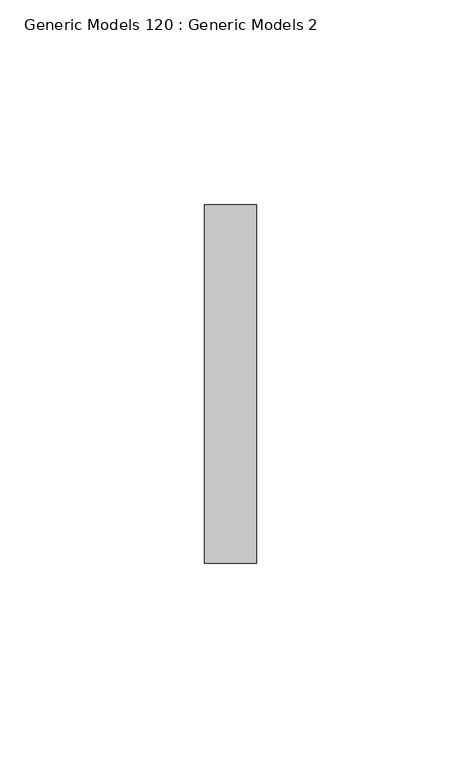
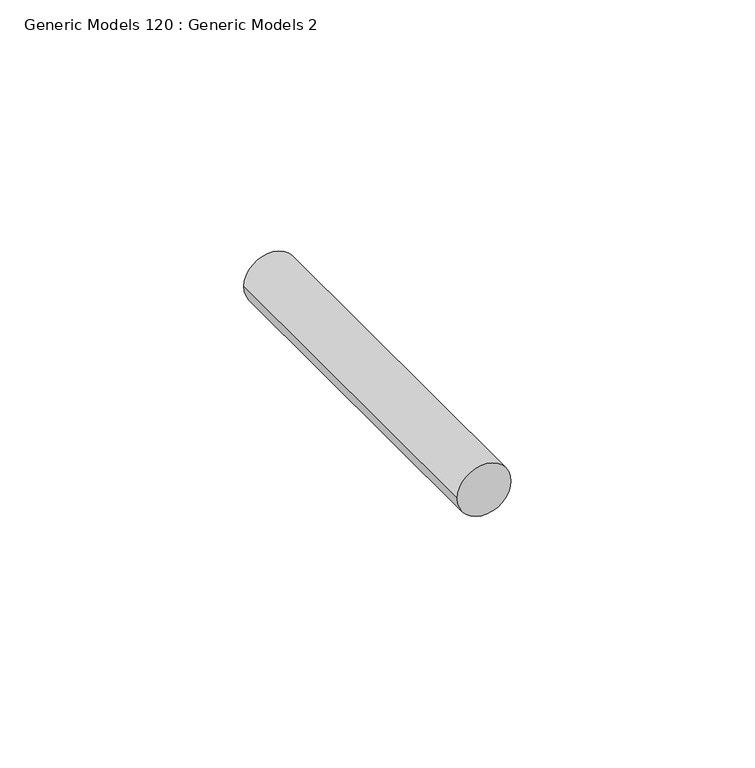
"""IFC4 building model written with IfcOpenShell, lengths in millimetres: proxy geometry, Generic Models 120 : Generic Models 2."""

import ifcopenshell
import ifcopenshell.guid

model = None  # the IFC model being written
_history = None  # IfcOwnerHistory: only IFC2X3 demands one
_inside = {}  # id of a spatial element -> (the spatial element, [elements in it])
_under = {}  # id of a project, library or spatial element -> (it, [spatial elements below it])
_declared = {}  # id of a project -> (the project, [libraries it declares])
_typed = {}  # id of a type object -> (the type object, [elements of that type])
_made_of = {}  # id of a material, layer set ... -> (it, [elements and type objects made of it])


def new_model(schema):
    """Start an empty IFC model of exactly this schema.

    Asked for "IFC4X3", IfcOpenShell would pick the latest addendum, in which some entities
    have other attributes; the version numbers below select the first issue.
    IFC2X3 requires an IfcOwnerHistory on every rooted entity: one is made here for all.
    """
    global model, _history
    if schema == "IFC4X3":
        model = ifcopenshell.file(schema_version=(4, 3, 0, 0))
    else:
        model = ifcopenshell.file(schema=schema)
    _inside.clear()
    _under.clear()
    _declared.clear()
    _typed.clear()
    _made_of.clear()
    _history = None
    if model.schema == "IFC2X3":
        org = make("IfcOrganization", Name="unknown")
        user = make(
            "IfcPersonAndOrganization",
            ThePerson=make("IfcPerson", FamilyName="unknown"),
            TheOrganization=org,
        )
        app = make(
            "IfcApplication",
            ApplicationDeveloper=org,
            Version="unknown",
            ApplicationFullName="unknown",
            ApplicationIdentifier="unknown",
        )
        _history = make(
            "IfcOwnerHistory",
            OwningUser=user,
            OwningApplication=app,
            ChangeAction="ADDED",
            CreationDate=0,
        )
    return model


def make(cls, **values):
    """One entity of the class cls with the attributes given. An attribute that is None is left unset."""
    return model.create_entity(
        cls, **{name: value for name, value in values.items() if value is not None}
    )


def rooted(cls, **values):
    """An entity with a GlobalId (a new one), such as an element, a storey or a relation."""
    return make(cls, GlobalId=ifcopenshell.guid.new(), OwnerHistory=_history, **values)


def si_unit(unit_type, name, prefix=None):
    """IfcSIUnit, for example si_unit("LENGTHUNIT", "METRE", prefix="MILLI")."""
    return make("IfcSIUnit", UnitType=unit_type, Prefix=prefix, Name=name)


def assignment(units):
    """IfcUnitAssignment: the units of a project."""
    return None if units is None else make("IfcUnitAssignment", Units=units)


def point(xyz):
    """IfcCartesianPoint."""
    return None if xyz is None else make("IfcCartesianPoint", Coordinates=xyz)


def direction(xyz):
    """IfcDirection."""
    return None if xyz is None else make("IfcDirection", DirectionRatios=xyz)


def frame(location, z_axis=None, x_axis=None):
    """IfcAxis2Placement3D, a coordinate frame: its origin and axes. An axis left out is left unset."""
    return make(
        "IfcAxis2Placement3D",
        Location=point(location),
        Axis=direction(z_axis),
        RefDirection=direction(x_axis),
    )


def frame_2d(location, x_axis=None):
    """IfcAxis2Placement2D, a coordinate frame in the plane: its origin and x axis."""
    return make(
        "IfcAxis2Placement2D", Location=point(location), RefDirection=direction(x_axis)
    )


def origin():
    """The frame at (0, 0, 0) with its axes left unset."""
    return frame((0.0, 0.0, 0.0))


def place(relative_to, where):
    """IfcLocalPlacement: puts the frame where relative to a parent placement (None: the world)."""
    return make(
        "IfcLocalPlacement", PlacementRelTo=relative_to, RelativePlacement=where
    )


def context(
    kind, dimensions, precision=None, world=None, true_north=None, identifier=None
):
    """IfcGeometricRepresentationContext, for example the 3D "Model" context."""
    return make(
        "IfcGeometricRepresentationContext",
        ContextIdentifier=identifier,
        ContextType=kind,
        CoordinateSpaceDimension=dimensions,
        Precision=precision,
        WorldCoordinateSystem=world,
        TrueNorth=true_north,
    )


def project(units=None, contexts=None):
    """IfcProject with its units and contexts."""
    return rooted(
        "IfcProject",
        Name="project",
        RepresentationContexts=contexts,
        UnitsInContext=assignment(units),
    )


def spatial(cls, under=None, at=None, **own):
    """A site, building, storey or space (cls), placed at a placement, below another one or the project."""
    s = rooted(cls, ObjectPlacement=at, **own)
    if under is not None:
        _under.setdefault(under.id(), (under, []))[1].append(s)
    return s


def circle_curve(where, radius):
    """IfcCircle in the frame where."""
    return make("IfcCircle", Position=where, Radius=radius)


def trimmed(basis, trim1, trim2, sense, master):
    """IfcTrimmedCurve: the piece of a basis curve between two trims."""
    return make(
        "IfcTrimmedCurve",
        BasisCurve=basis,
        Trim1=trim1,
        Trim2=trim2,
        SenseAgreement=sense,
        MasterRepresentation=master,
    )


def segment(curve, same_sense, transition):
    """IfcCompositeCurveSegment."""
    return make(
        "IfcCompositeCurveSegment",
        Transition=transition,
        SameSense=same_sense,
        ParentCurve=curve,
    )


def composite_curve(segments, self_intersect=None):
    """IfcCompositeCurve: segments joined end to end."""
    return make("IfcCompositeCurve", Segments=segments, SelfIntersect=self_intersect)


def outline(outer, holes=None, kind="AREA"):
    """IfcArbitraryClosedProfileDef: a profile drawn as a closed curve; with holes, ...WithVoids."""
    if holes is None:
        return make("IfcArbitraryClosedProfileDef", ProfileType=kind, OuterCurve=outer)
    return make(
        "IfcArbitraryProfileDefWithVoids",
        ProfileType=kind,
        OuterCurve=outer,
        InnerCurves=holes,
    )


def extrude(swept, where, along, depth):
    """IfcExtrudedAreaSolid: the profile swept, set in the frame where, extruded along a direction by depth."""
    return make(
        "IfcExtrudedAreaSolid",
        SweptArea=swept,
        Position=where,
        ExtrudedDirection=direction(along),
        Depth=depth,
    )


def shape(context_of_items, identifier, shape_type, items):
    """IfcShapeRepresentation: the items that make up one representation, for example the "Body"."""
    return make(
        "IfcShapeRepresentation",
        ContextOfItems=context_of_items,
        RepresentationIdentifier=identifier,
        RepresentationType=shape_type,
        Items=items,
    )


def source(mapping_origin, context_of_items, identifier, shape_type, items):
    """IfcRepresentationMap: a shape defined once, which mapped items show again and again."""
    return make(
        "IfcRepresentationMap",
        MappingOrigin=mapping_origin,
        MappedRepresentation=shape(context_of_items, identifier, shape_type, items),
    )


def transform(
    local_origin,
    x_axis=None,
    y_axis=None,
    z_axis=None,
    scale=None,
    scale2=None,
    scale3=None,
    uniform=True,
):
    """IfcCartesianTransformationOperator3D, or its non-uniform kind. x_axis, y_axis, z_axis: its Axis1, 2, 3."""
    if uniform:
        return make(
            "IfcCartesianTransformationOperator3D",
            Axis1=direction(x_axis),
            Axis2=direction(y_axis),
            LocalOrigin=point(local_origin),
            Scale=scale,
            Axis3=direction(z_axis),
        )
    return make(
        "IfcCartesianTransformationOperator3DnonUniform",
        Axis1=direction(x_axis),
        Axis2=direction(y_axis),
        LocalOrigin=point(local_origin),
        Scale=scale,
        Axis3=direction(z_axis),
        Scale2=scale2,
        Scale3=scale3,
    )


def mapped(mapping_source, mapping_target):
    """IfcMappedItem: shows the shape of a source again, moved by a transform."""
    return make(
        "IfcMappedItem", MappingSource=mapping_source, MappingTarget=mapping_target
    )


def made_of(thing, what):
    """Note that an element or type object is made of a material, layer set ...; save() writes the relation."""
    if what is not None:
        _made_of.setdefault(what.id(), (what, []))[1].append(thing)
    return thing


def element(
    cls,
    number,
    at=None,
    inside=None,
    cuts=None,
    type_object=None,
    material=None,
    context=None,
    identifier="Body",
    shape_type=None,
    held_by="IfcProductDefinitionShape",
    body=None,
    shapes=None,
    **own,
):
    """One element of the class cls, such as IfcWall. Its Tag is "e" and its number.

    at: its placement. inside: the storey or other place that contains it. cuts: it is an
    opening in that element (IfcRelVoidsElement). A single representation is given by context,
    identifier, shape_type and body (its items); several are given by shapes. held_by: the class
    of the entity that holds the representations. save() writes the other relations.
    """
    e = rooted(cls, Tag="e%d" % number, ObjectPlacement=at, **own)
    if body is not None:
        shapes = [shape(context, identifier, shape_type, body)]
    if shapes is not None:
        e.Representation = make(held_by, Representations=shapes)
    if inside is not None:
        _inside.setdefault(inside.id(), (inside, []))[1].append(e)
    if cuts is not None:
        rooted(
            "IfcRelVoidsElement", RelatingBuildingElement=cuts, RelatedOpeningElement=e
        )
    if type_object is not None:
        _typed.setdefault(type_object.id(), (type_object, []))[1].append(e)
    return made_of(e, material)


def aggregate(whole, parts):
    """IfcRelAggregates: a whole, such as a stair, and the parts it consists of."""
    return rooted("IfcRelAggregates", RelatingObject=whole, RelatedObjects=parts)


def save(model, path):
    """Write the relations noted so far, then the file.

    IfcRelAggregates (storeys below a building ...), IfcRelContainedInSpatialStructure (elements
    in a storey), IfcRelDefinesByType, IfcRelAssociatesMaterial and IfcRelDeclares: one each for
    every whole, place, type object, material and project.
    """
    for whole, parts in _under.values():
        aggregate(whole, parts)
    for where, things in _inside.values():
        rooted(
            "IfcRelContainedInSpatialStructure",
            RelatedElements=things,
            RelatingStructure=where,
        )
    for kind, things in _typed.values():
        rooted("IfcRelDefinesByType", RelatedObjects=things, RelatingType=kind)
    for what, things in _made_of.values():
        rooted("IfcRelAssociatesMaterial", RelatedObjects=things, RelatingMaterial=what)
    for by, libraries in _declared.values():
        rooted("IfcRelDeclares", RelatingContext=by, RelatedDefinitions=libraries)
    model.write(path)


def generic_models_120_generic_models_2_17b25060(model_context):
    return source(origin(), model_context, "Body", "SweptSolid", [
        extrude(outline(composite_curve([segment(trimmed(circle_curve(frame_2d((38031.9291136, 7018.1346014)), 6.35), [point((38031.9291136, 7024.4846014))], [point((38031.9291136, 7011.7846014))], False, "CARTESIAN"), True, "CONTINUOUS"), segment(trimmed(circle_curve(frame_2d((38031.9291136, 7018.1346014)), 6.35), [point((38031.9291136, 7011.7846014))], [point((38031.9291136, 7024.4846014))], False, "CARTESIAN"), True, "CONTINUOUS")], self_intersect=False)), frame((0.0, 1848.3666731, 0.0), z_axis=(0.0, 1.0, 0.0), x_axis=(0.0, 0.0, 1.0)), (0.0, 0.0, 1.0), 87.551022),
    ])


if __name__ == "__main__":
    model = new_model("IFC4")
    model_context = context("Model", 3, world=origin())
    ifc_project = project(units=[si_unit("LENGTHUNIT", "METRE", prefix="MILLI")], contexts=[model_context])
    site = spatial("IfcSite", under=ifc_project)
    building = spatial("IfcBuilding", under=site)
    placement = place(None, origin())
    generic_models_120_generic_models_2_shape = generic_models_120_generic_models_2_17b25060(model_context)
    element("IfcBuildingElementProxy", 1, Name="Generic Models 120 : Generic Models 2", ObjectType="Generic Models 120 : Generic Models 2", at=placement, inside=building, context=model_context, shape_type="MappedRepresentation", body=[
        mapped(generic_models_120_generic_models_2_shape, transform((0.0, 0.0, 0.0), x_axis=(1.0, 0.0, 0.0), y_axis=(0.0, 1.0, 0.0), z_axis=(0.0, 0.0, 1.0))),
    ])
    save(model, "model.ifc")

# Revit data of these elements
# Element 1 (IfcBuildingElementProxy, "Generic Models 120 : Generic Models 2")
#   Materials on its faces: "S.S. LAG BOLT - SEE STRUCT. DWGS"
# Materials
#   "S.S. LAG BOLT - SEE STRUCT. DWGS": class "Generic", colour RGB 120 120 120, transparency 0, Cost = 0
